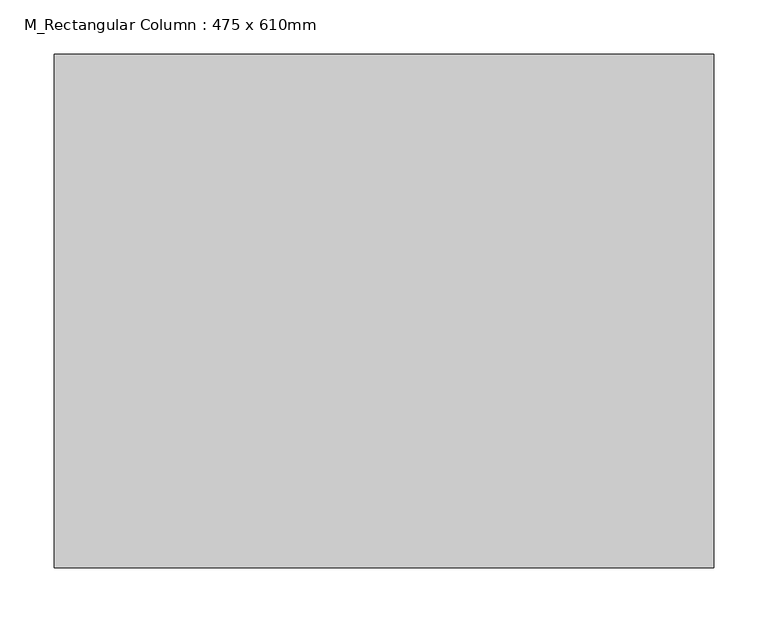
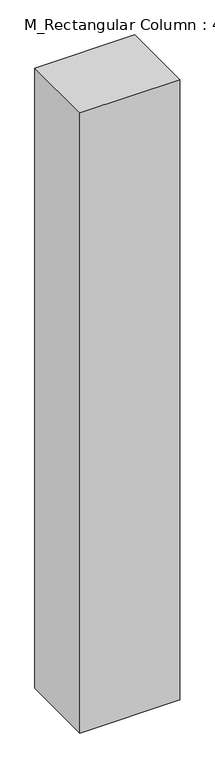
"""IFC4 building model written with IfcOpenShell, lengths in millimetres: column geometry, M_Rectangular Column : 475 x 610mm."""

from ifc_helpers import new_model, si_unit, frame, origin, place, context, project, spatial, polyline, outline, extrude, source, transform, mapped, element, save


def m_rectangular_column_475_x_610mm_1e9c0db0(model_context):
    return source(origin(), model_context, "Body", "SweptSolid", [
        extrude(outline(polyline([(305.0, 237.5), (305.0, -237.5), (-305.0, -237.5), (-305.0, 237.5), (305.0, 237.5)])), frame((0.0, 0.0, -4000.0), z_axis=(0.0, 0.0, 1.0), x_axis=(1.0, 0.0, 0.0)), (0.0, 0.0, 1.0), 4000.0),
    ])


if __name__ == "__main__":
    model = new_model("IFC4")
    model_context = context("Model", 3, world=origin())
    ifc_project = project(units=[si_unit("LENGTHUNIT", "METRE", prefix="MILLI")], contexts=[model_context])
    site = spatial("IfcSite", under=ifc_project)
    building = spatial("IfcBuilding", under=site)
    placement = place(None, origin())
    m_rectangular_column_475_x_610mm_shape = m_rectangular_column_475_x_610mm_1e9c0db0(model_context)
    element("IfcColumn", 1, ObjectType="M_Rectangular Column : 475 x 610mm", at=placement, inside=building, context=model_context, shape_type="MappedRepresentation", body=[
        mapped(m_rectangular_column_475_x_610mm_shape, transform((0.0, 0.0, 0.0), x_axis=(1.0, 0.0, 0.0), y_axis=(0.0, 1.0, 0.0), z_axis=(0.0, 0.0, 1.0))),
    ])
    save(model, "model.ifc")

# Revit data of these elements
# Type "M_Rectangular Column : 475 x 610mm"
#   Depth = 475 mm
#   Offset Base = 0 mm
#   Offset Top = 0 mm
#   Width = 610 mm
#   Material = Copper
# Element 1 (IfcColumn, "M_Rectangular Column : 475 x 610mm")
#   Materials on its faces: "Copper"
# Materials
#   "Copper": class "Metal", colour RGB 0 0 0, transparency 0, Description = "Copper, matte finish", Cost = 0
